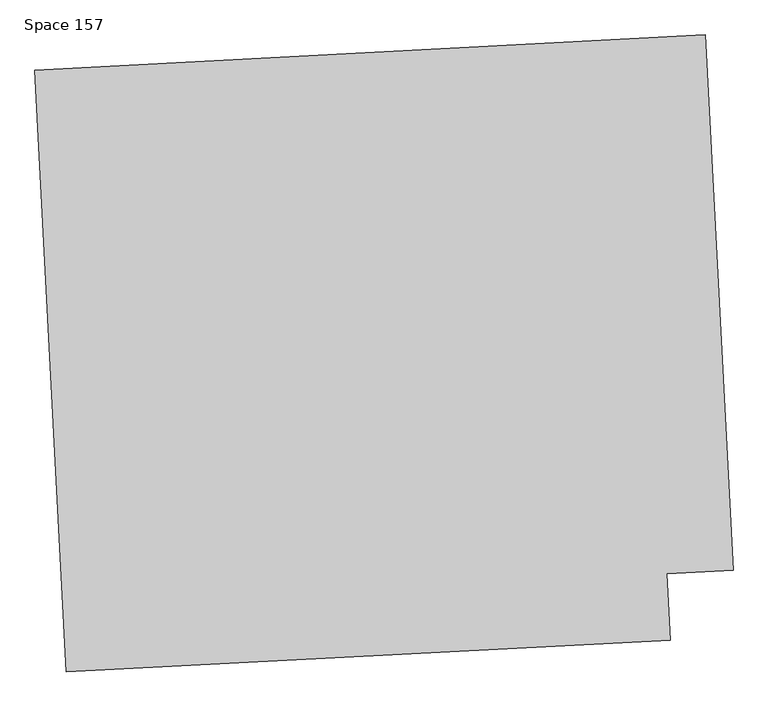
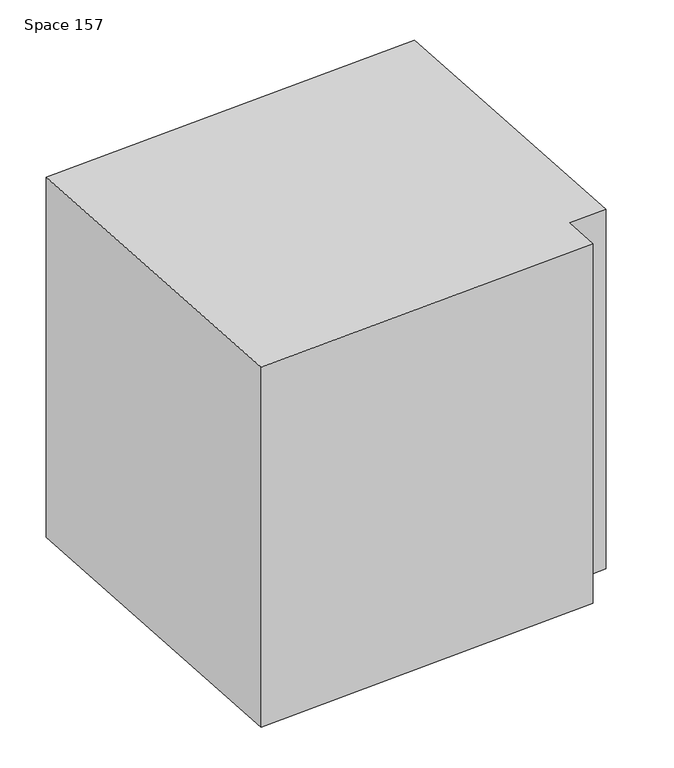
"""IFC4 building model written with IfcOpenShell, lengths in millimetres: proxy geometry, Space 157."""

from ifc_helpers import new_model, si_unit, frame, origin, place, context, project, spatial, polyline, outline, extrude, source, transform, mapped, element, save


def space_157_51e8f62b(model_context):
    return source(origin(), model_context, "Body", "SweptSolid", [
        extrude(outline(polyline([(12839.1348701, -34556.7556259), (12695.8992082, -31823.6563837), (15739.7220301, -31664.1363891), (15867.1718592, -34096.0239978), (15565.9602258, -34111.8098306), (15581.7460586, -34413.0214641), (12839.1348701, -34556.7556259)])), frame((0.0, 0.0, 3810.0), z_axis=(0.0, 0.0, 1.0), x_axis=(1.0, 0.0, 0.0)), (0.0, 0.0, 1.0), 3048.0),
    ])


if __name__ == "__main__":
    model = new_model("IFC4")
    model_context = context("Model", 3, world=origin())
    ifc_project = project(units=[si_unit("LENGTHUNIT", "METRE", prefix="MILLI")], contexts=[model_context])
    site = spatial("IfcSite", under=ifc_project)
    building = spatial("IfcBuilding", under=site)
    placement = place(None, origin())
    space_157_shape = space_157_51e8f62b(model_context)
    element("IfcBuildingElementProxy", 1, Name="Space 157", ObjectType="Space 157", at=placement, inside=building, context=model_context, shape_type="MappedRepresentation", body=[
        mapped(space_157_shape, transform((0.0, 0.0, 0.0), x_axis=(1.0, 0.0, 0.0), y_axis=(0.0, 1.0, 0.0), z_axis=(0.0, 0.0, 1.0))),
    ])
    save(model, "model.ifc")

# Revit data of these elements
# Element 1 (IfcBuildingElementProxy, "Space 157")
#   Materials on its faces: "Render Material 255-255-255"
# Materials
#   "Render Material 255-255-255": class "Unassigned", colour RGB 255 255 255, transparency 0
